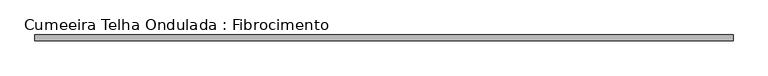
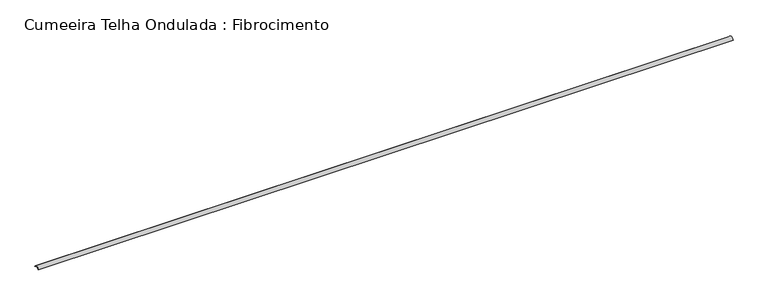
"""IFC4 building model written with IfcOpenShell, lengths in millimetres: beam geometry, Cumeeira Telha Ondulada : Fibrocimento."""

import ifcopenshell
import ifcopenshell.guid

model = None  # the IFC model being written
_history = None  # IfcOwnerHistory: only IFC2X3 demands one
_inside = {}  # id of a spatial element -> (the spatial element, [elements in it])
_under = {}  # id of a project, library or spatial element -> (it, [spatial elements below it])
_declared = {}  # id of a project -> (the project, [libraries it declares])
_typed = {}  # id of a type object -> (the type object, [elements of that type])
_made_of = {}  # id of a material, layer set ... -> (it, [elements and type objects made of it])


def new_model(schema):
    """Start an empty IFC model of exactly this schema.

    Asked for "IFC4X3", IfcOpenShell would pick the latest addendum, in which some entities
    have other attributes; the version numbers below select the first issue.
    IFC2X3 requires an IfcOwnerHistory on every rooted entity: one is made here for all.
    """
    global model, _history
    if schema == "IFC4X3":
        model = ifcopenshell.file(schema_version=(4, 3, 0, 0))
    else:
        model = ifcopenshell.file(schema=schema)
    _inside.clear()
    _under.clear()
    _declared.clear()
    _typed.clear()
    _made_of.clear()
    _history = None
    if model.schema == "IFC2X3":
        org = make("IfcOrganization", Name="unknown")
        user = make(
            "IfcPersonAndOrganization",
            ThePerson=make("IfcPerson", FamilyName="unknown"),
            TheOrganization=org,
        )
        app = make(
            "IfcApplication",
            ApplicationDeveloper=org,
            Version="unknown",
            ApplicationFullName="unknown",
            ApplicationIdentifier="unknown",
        )
        _history = make(
            "IfcOwnerHistory",
            OwningUser=user,
            OwningApplication=app,
            ChangeAction="ADDED",
            CreationDate=0,
        )
    return model


def make(cls, **values):
    """One entity of the class cls with the attributes given. An attribute that is None is left unset."""
    return model.create_entity(
        cls, **{name: value for name, value in values.items() if value is not None}
    )


def rooted(cls, **values):
    """An entity with a GlobalId (a new one), such as an element, a storey or a relation."""
    return make(cls, GlobalId=ifcopenshell.guid.new(), OwnerHistory=_history, **values)


def si_unit(unit_type, name, prefix=None):
    """IfcSIUnit, for example si_unit("LENGTHUNIT", "METRE", prefix="MILLI")."""
    return make("IfcSIUnit", UnitType=unit_type, Prefix=prefix, Name=name)


def assignment(units):
    """IfcUnitAssignment: the units of a project."""
    return None if units is None else make("IfcUnitAssignment", Units=units)


def point(xyz):
    """IfcCartesianPoint."""
    return None if xyz is None else make("IfcCartesianPoint", Coordinates=xyz)


def direction(xyz):
    """IfcDirection."""
    return None if xyz is None else make("IfcDirection", DirectionRatios=xyz)


def frame(location, z_axis=None, x_axis=None):
    """IfcAxis2Placement3D, a coordinate frame: its origin and axes. An axis left out is left unset."""
    return make(
        "IfcAxis2Placement3D",
        Location=point(location),
        Axis=direction(z_axis),
        RefDirection=direction(x_axis),
    )


def frame_2d(location, x_axis=None):
    """IfcAxis2Placement2D, a coordinate frame in the plane: its origin and x axis."""
    return make(
        "IfcAxis2Placement2D", Location=point(location), RefDirection=direction(x_axis)
    )


def origin():
    """The frame at (0, 0, 0) with its axes left unset."""
    return frame((0.0, 0.0, 0.0))


def place(relative_to, where):
    """IfcLocalPlacement: puts the frame where relative to a parent placement (None: the world)."""
    return make(
        "IfcLocalPlacement", PlacementRelTo=relative_to, RelativePlacement=where
    )


def context(
    kind, dimensions, precision=None, world=None, true_north=None, identifier=None
):
    """IfcGeometricRepresentationContext, for example the 3D "Model" context."""
    return make(
        "IfcGeometricRepresentationContext",
        ContextIdentifier=identifier,
        ContextType=kind,
        CoordinateSpaceDimension=dimensions,
        Precision=precision,
        WorldCoordinateSystem=world,
        TrueNorth=true_north,
    )


def project(units=None, contexts=None):
    """IfcProject with its units and contexts."""
    return rooted(
        "IfcProject",
        Name="project",
        RepresentationContexts=contexts,
        UnitsInContext=assignment(units),
    )


def spatial(cls, under=None, at=None, **own):
    """A site, building, storey or space (cls), placed at a placement, below another one or the project."""
    s = rooted(cls, ObjectPlacement=at, **own)
    if under is not None:
        _under.setdefault(under.id(), (under, []))[1].append(s)
    return s


def polyline(points):
    """IfcPolyline through the points."""
    return make("IfcPolyline", Points=[point(p) for p in points])


def circle_curve(where, radius):
    """IfcCircle in the frame where."""
    return make("IfcCircle", Position=where, Radius=radius)


def trimmed(basis, trim1, trim2, sense, master):
    """IfcTrimmedCurve: the piece of a basis curve between two trims."""
    return make(
        "IfcTrimmedCurve",
        BasisCurve=basis,
        Trim1=trim1,
        Trim2=trim2,
        SenseAgreement=sense,
        MasterRepresentation=master,
    )


def segment(curve, same_sense, transition):
    """IfcCompositeCurveSegment."""
    return make(
        "IfcCompositeCurveSegment",
        Transition=transition,
        SameSense=same_sense,
        ParentCurve=curve,
    )


def composite_curve(segments, self_intersect=None):
    """IfcCompositeCurve: segments joined end to end."""
    return make("IfcCompositeCurve", Segments=segments, SelfIntersect=self_intersect)


def outline(outer, holes=None, kind="AREA"):
    """IfcArbitraryClosedProfileDef: a profile drawn as a closed curve; with holes, ...WithVoids."""
    if holes is None:
        return make("IfcArbitraryClosedProfileDef", ProfileType=kind, OuterCurve=outer)
    return make(
        "IfcArbitraryProfileDefWithVoids",
        ProfileType=kind,
        OuterCurve=outer,
        InnerCurves=holes,
    )


def extrude(swept, where, along, depth):
    """IfcExtrudedAreaSolid: the profile swept, set in the frame where, extruded along a direction by depth."""
    return make(
        "IfcExtrudedAreaSolid",
        SweptArea=swept,
        Position=where,
        ExtrudedDirection=direction(along),
        Depth=depth,
    )


def shape(context_of_items, identifier, shape_type, items):
    """IfcShapeRepresentation: the items that make up one representation, for example the "Body"."""
    return make(
        "IfcShapeRepresentation",
        ContextOfItems=context_of_items,
        RepresentationIdentifier=identifier,
        RepresentationType=shape_type,
        Items=items,
    )


def source(mapping_origin, context_of_items, identifier, shape_type, items):
    """IfcRepresentationMap: a shape defined once, which mapped items show again and again."""
    return make(
        "IfcRepresentationMap",
        MappingOrigin=mapping_origin,
        MappedRepresentation=shape(context_of_items, identifier, shape_type, items),
    )


def transform(
    local_origin,
    x_axis=None,
    y_axis=None,
    z_axis=None,
    scale=None,
    scale2=None,
    scale3=None,
    uniform=True,
):
    """IfcCartesianTransformationOperator3D, or its non-uniform kind. x_axis, y_axis, z_axis: its Axis1, 2, 3."""
    if uniform:
        return make(
            "IfcCartesianTransformationOperator3D",
            Axis1=direction(x_axis),
            Axis2=direction(y_axis),
            LocalOrigin=point(local_origin),
            Scale=scale,
            Axis3=direction(z_axis),
        )
    return make(
        "IfcCartesianTransformationOperator3DnonUniform",
        Axis1=direction(x_axis),
        Axis2=direction(y_axis),
        LocalOrigin=point(local_origin),
        Scale=scale,
        Axis3=direction(z_axis),
        Scale2=scale2,
        Scale3=scale3,
    )


def mapped(mapping_source, mapping_target):
    """IfcMappedItem: shows the shape of a source again, moved by a transform."""
    return make(
        "IfcMappedItem", MappingSource=mapping_source, MappingTarget=mapping_target
    )


def made_of(thing, what):
    """Note that an element or type object is made of a material, layer set ...; save() writes the relation."""
    if what is not None:
        _made_of.setdefault(what.id(), (what, []))[1].append(thing)
    return thing


def element(
    cls,
    number,
    at=None,
    inside=None,
    cuts=None,
    type_object=None,
    material=None,
    context=None,
    identifier="Body",
    shape_type=None,
    held_by="IfcProductDefinitionShape",
    body=None,
    shapes=None,
    **own,
):
    """One element of the class cls, such as IfcWall. Its Tag is "e" and its number.

    at: its placement. inside: the storey or other place that contains it. cuts: it is an
    opening in that element (IfcRelVoidsElement). A single representation is given by context,
    identifier, shape_type and body (its items); several are given by shapes. held_by: the class
    of the entity that holds the representations. save() writes the other relations.
    """
    e = rooted(cls, Tag="e%d" % number, ObjectPlacement=at, **own)
    if body is not None:
        shapes = [shape(context, identifier, shape_type, body)]
    if shapes is not None:
        e.Representation = make(held_by, Representations=shapes)
    if inside is not None:
        _inside.setdefault(inside.id(), (inside, []))[1].append(e)
    if cuts is not None:
        rooted(
            "IfcRelVoidsElement", RelatingBuildingElement=cuts, RelatedOpeningElement=e
        )
    if type_object is not None:
        _typed.setdefault(type_object.id(), (type_object, []))[1].append(e)
    return made_of(e, material)


def aggregate(whole, parts):
    """IfcRelAggregates: a whole, such as a stair, and the parts it consists of."""
    return rooted("IfcRelAggregates", RelatingObject=whole, RelatedObjects=parts)


def save(model, path):
    """Write the relations noted so far, then the file.

    IfcRelAggregates (storeys below a building ...), IfcRelContainedInSpatialStructure (elements
    in a storey), IfcRelDefinesByType, IfcRelAssociatesMaterial and IfcRelDeclares: one each for
    every whole, place, type object, material and project.
    """
    for whole, parts in _under.values():
        aggregate(whole, parts)
    for where, things in _inside.values():
        rooted(
            "IfcRelContainedInSpatialStructure",
            RelatedElements=things,
            RelatingStructure=where,
        )
    for kind, things in _typed.values():
        rooted("IfcRelDefinesByType", RelatedObjects=things, RelatingType=kind)
    for what, things in _made_of.values():
        rooted("IfcRelAssociatesMaterial", RelatedObjects=things, RelatingMaterial=what)
    for by, libraries in _declared.values():
        rooted("IfcRelDeclares", RelatingContext=by, RelatedDefinitions=libraries)
    model.write(path)


def cumeeira_telha_ondulada_fibrocimento_80a8fd81(model_context):
    return source(origin(), model_context, "Body", "SweptSolid", [
        extrude(outline(composite_curve([segment(polyline([(58.3970135, 42.4437972), (53.9055884, 40.2467307)]), True, "CONTINUOUS"), segment(trimmed(circle_curve(frame_2d((-1.6029865, 13.0936483)), 61.7939461), [point((53.9055884, 40.2467307))], [point((-57.1115615, 40.2467307))], True, "CARTESIAN"), True, "CONTINUOUS"), segment(polyline([(-57.1115615, 40.2467307), (-61.6029865, 42.4437972)]), True, "CONTINUOUS"), segment(trimmed(circle_curve(frame_2d((-1.6029865, 13.0936483)), 66.7939461), [point((-61.6029865, 42.4437972))], [point((58.3970135, 42.4437972))], False, "CARTESIAN"), True, "CONTINUOUS")], self_intersect=False)), frame((-7085.3584094, 0.0, 0.0), z_axis=(1.0, 0.0, 0.0), x_axis=(0.0, 1.0, 0.0)), (0.0, 0.0, 1.0), 14170.7168187),
    ])


if __name__ == "__main__":
    model = new_model("IFC4")
    model_context = context("Model", 3, world=origin())
    ifc_project = project(units=[si_unit("LENGTHUNIT", "METRE", prefix="MILLI")], contexts=[model_context])
    site = spatial("IfcSite", under=ifc_project)
    building = spatial("IfcBuilding", under=site)
    placement = place(None, origin())
    cumeeira_telha_ondulada_fibrocimento_shape = cumeeira_telha_ondulada_fibrocimento_80a8fd81(model_context)
    element("IfcBeam", 1, ObjectType="Cumeeira Telha Ondulada : Fibrocimento", at=placement, inside=building, context=model_context, shape_type="MappedRepresentation", body=[
        mapped(cumeeira_telha_ondulada_fibrocimento_shape, transform((0.0, 0.0, 0.0), x_axis=(1.0, 0.0, 0.0), y_axis=(0.0, 1.0, 0.0), z_axis=(0.0, 0.0, 1.0))),
    ])
    save(model, "model.ifc")

# Revit data of these elements
# Type "Cumeeira Telha Ondulada : Fibrocimento"
#   Cost = 5
#   Length [instance default] = 1.524 m
#   b = 0.07 m
#   h = 0.16 m
#   Structural Material = .TELHA DE FIBROCIMENTO
#   Assembly Code = ""
# Element 1 (IfcBeam, "Cumeeira Telha Ondulada : Fibrocimento")
#   Materials on its faces: ".TELHA DE FIBROCIMENTO"
# Materials
#   ".TELHA DE FIBROCIMENTO": class "CC_TELHADO", colour RGB 77 77 76, transparency 0, Description = "TELHA ONDULADA FIBROCIMENTO", Cost = 0
